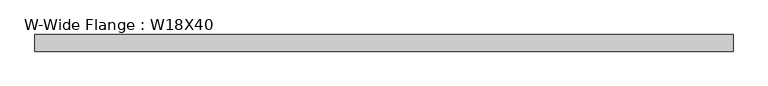
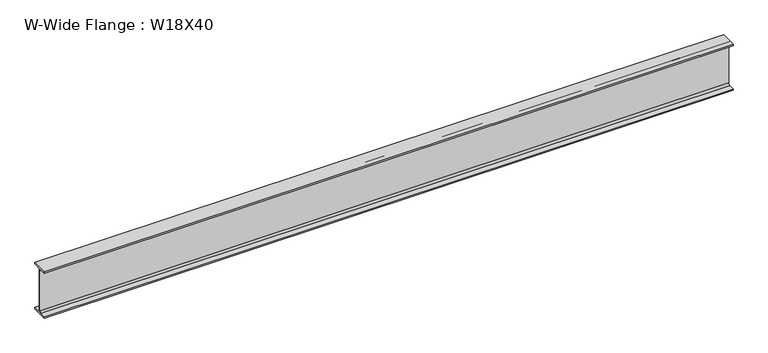
"""IFC4 building model written with IfcOpenShell, lengths in millimetres: beam geometry, W-Wide Flange : W18X40."""

import ifcopenshell
import ifcopenshell.guid

model = None  # the IFC model being written
_history = None  # IfcOwnerHistory: only IFC2X3 demands one
_inside = {}  # id of a spatial element -> (the spatial element, [elements in it])
_under = {}  # id of a project, library or spatial element -> (it, [spatial elements below it])
_declared = {}  # id of a project -> (the project, [libraries it declares])
_typed = {}  # id of a type object -> (the type object, [elements of that type])
_made_of = {}  # id of a material, layer set ... -> (it, [elements and type objects made of it])


def new_model(schema):
    """Start an empty IFC model of exactly this schema.

    Asked for "IFC4X3", IfcOpenShell would pick the latest addendum, in which some entities
    have other attributes; the version numbers below select the first issue.
    IFC2X3 requires an IfcOwnerHistory on every rooted entity: one is made here for all.
    """
    global model, _history
    if schema == "IFC4X3":
        model = ifcopenshell.file(schema_version=(4, 3, 0, 0))
    else:
        model = ifcopenshell.file(schema=schema)
    _inside.clear()
    _under.clear()
    _declared.clear()
    _typed.clear()
    _made_of.clear()
    _history = None
    if model.schema == "IFC2X3":
        org = make("IfcOrganization", Name="unknown")
        user = make(
            "IfcPersonAndOrganization",
            ThePerson=make("IfcPerson", FamilyName="unknown"),
            TheOrganization=org,
        )
        app = make(
            "IfcApplication",
            ApplicationDeveloper=org,
            Version="unknown",
            ApplicationFullName="unknown",
            ApplicationIdentifier="unknown",
        )
        _history = make(
            "IfcOwnerHistory",
            OwningUser=user,
            OwningApplication=app,
            ChangeAction="ADDED",
            CreationDate=0,
        )
    return model


def make(cls, **values):
    """One entity of the class cls with the attributes given. An attribute that is None is left unset."""
    return model.create_entity(
        cls, **{name: value for name, value in values.items() if value is not None}
    )


def rooted(cls, **values):
    """An entity with a GlobalId (a new one), such as an element, a storey or a relation."""
    return make(cls, GlobalId=ifcopenshell.guid.new(), OwnerHistory=_history, **values)


def si_unit(unit_type, name, prefix=None):
    """IfcSIUnit, for example si_unit("LENGTHUNIT", "METRE", prefix="MILLI")."""
    return make("IfcSIUnit", UnitType=unit_type, Prefix=prefix, Name=name)


def assignment(units):
    """IfcUnitAssignment: the units of a project."""
    return None if units is None else make("IfcUnitAssignment", Units=units)


def point(xyz):
    """IfcCartesianPoint."""
    return None if xyz is None else make("IfcCartesianPoint", Coordinates=xyz)


def direction(xyz):
    """IfcDirection."""
    return None if xyz is None else make("IfcDirection", DirectionRatios=xyz)


def frame(location, z_axis=None, x_axis=None):
    """IfcAxis2Placement3D, a coordinate frame: its origin and axes. An axis left out is left unset."""
    return make(
        "IfcAxis2Placement3D",
        Location=point(location),
        Axis=direction(z_axis),
        RefDirection=direction(x_axis),
    )


def frame_2d(location, x_axis=None):
    """IfcAxis2Placement2D, a coordinate frame in the plane: its origin and x axis."""
    return make(
        "IfcAxis2Placement2D", Location=point(location), RefDirection=direction(x_axis)
    )


def origin():
    """The frame at (0, 0, 0) with its axes left unset."""
    return frame((0.0, 0.0, 0.0))


def place(relative_to, where):
    """IfcLocalPlacement: puts the frame where relative to a parent placement (None: the world)."""
    return make(
        "IfcLocalPlacement", PlacementRelTo=relative_to, RelativePlacement=where
    )


def context(
    kind, dimensions, precision=None, world=None, true_north=None, identifier=None
):
    """IfcGeometricRepresentationContext, for example the 3D "Model" context."""
    return make(
        "IfcGeometricRepresentationContext",
        ContextIdentifier=identifier,
        ContextType=kind,
        CoordinateSpaceDimension=dimensions,
        Precision=precision,
        WorldCoordinateSystem=world,
        TrueNorth=true_north,
    )


def project(units=None, contexts=None):
    """IfcProject with its units and contexts."""
    return rooted(
        "IfcProject",
        Name="project",
        RepresentationContexts=contexts,
        UnitsInContext=assignment(units),
    )


def spatial(cls, under=None, at=None, **own):
    """A site, building, storey or space (cls), placed at a placement, below another one or the project."""
    s = rooted(cls, ObjectPlacement=at, **own)
    if under is not None:
        _under.setdefault(under.id(), (under, []))[1].append(s)
    return s


def polyline(points):
    """IfcPolyline through the points."""
    return make("IfcPolyline", Points=[point(p) for p in points])


def circle_curve(where, radius):
    """IfcCircle in the frame where."""
    return make("IfcCircle", Position=where, Radius=radius)


def trimmed(basis, trim1, trim2, sense, master):
    """IfcTrimmedCurve: the piece of a basis curve between two trims."""
    return make(
        "IfcTrimmedCurve",
        BasisCurve=basis,
        Trim1=trim1,
        Trim2=trim2,
        SenseAgreement=sense,
        MasterRepresentation=master,
    )


def segment(curve, same_sense, transition):
    """IfcCompositeCurveSegment."""
    return make(
        "IfcCompositeCurveSegment",
        Transition=transition,
        SameSense=same_sense,
        ParentCurve=curve,
    )


def composite_curve(segments, self_intersect=None):
    """IfcCompositeCurve: segments joined end to end."""
    return make("IfcCompositeCurve", Segments=segments, SelfIntersect=self_intersect)


def outline(outer, holes=None, kind="AREA"):
    """IfcArbitraryClosedProfileDef: a profile drawn as a closed curve; with holes, ...WithVoids."""
    if holes is None:
        return make("IfcArbitraryClosedProfileDef", ProfileType=kind, OuterCurve=outer)
    return make(
        "IfcArbitraryProfileDefWithVoids",
        ProfileType=kind,
        OuterCurve=outer,
        InnerCurves=holes,
    )


def extrude(swept, where, along, depth):
    """IfcExtrudedAreaSolid: the profile swept, set in the frame where, extruded along a direction by depth."""
    return make(
        "IfcExtrudedAreaSolid",
        SweptArea=swept,
        Position=where,
        ExtrudedDirection=direction(along),
        Depth=depth,
    )


def shape(context_of_items, identifier, shape_type, items):
    """IfcShapeRepresentation: the items that make up one representation, for example the "Body"."""
    return make(
        "IfcShapeRepresentation",
        ContextOfItems=context_of_items,
        RepresentationIdentifier=identifier,
        RepresentationType=shape_type,
        Items=items,
    )


def source(mapping_origin, context_of_items, identifier, shape_type, items):
    """IfcRepresentationMap: a shape defined once, which mapped items show again and again."""
    return make(
        "IfcRepresentationMap",
        MappingOrigin=mapping_origin,
        MappedRepresentation=shape(context_of_items, identifier, shape_type, items),
    )


def transform(
    local_origin,
    x_axis=None,
    y_axis=None,
    z_axis=None,
    scale=None,
    scale2=None,
    scale3=None,
    uniform=True,
):
    """IfcCartesianTransformationOperator3D, or its non-uniform kind. x_axis, y_axis, z_axis: its Axis1, 2, 3."""
    if uniform:
        return make(
            "IfcCartesianTransformationOperator3D",
            Axis1=direction(x_axis),
            Axis2=direction(y_axis),
            LocalOrigin=point(local_origin),
            Scale=scale,
            Axis3=direction(z_axis),
        )
    return make(
        "IfcCartesianTransformationOperator3DnonUniform",
        Axis1=direction(x_axis),
        Axis2=direction(y_axis),
        LocalOrigin=point(local_origin),
        Scale=scale,
        Axis3=direction(z_axis),
        Scale2=scale2,
        Scale3=scale3,
    )


def mapped(mapping_source, mapping_target):
    """IfcMappedItem: shows the shape of a source again, moved by a transform."""
    return make(
        "IfcMappedItem", MappingSource=mapping_source, MappingTarget=mapping_target
    )


def made_of(thing, what):
    """Note that an element or type object is made of a material, layer set ...; save() writes the relation."""
    if what is not None:
        _made_of.setdefault(what.id(), (what, []))[1].append(thing)
    return thing


def element(
    cls,
    number,
    at=None,
    inside=None,
    cuts=None,
    type_object=None,
    material=None,
    context=None,
    identifier="Body",
    shape_type=None,
    held_by="IfcProductDefinitionShape",
    body=None,
    shapes=None,
    **own,
):
    """One element of the class cls, such as IfcWall. Its Tag is "e" and its number.

    at: its placement. inside: the storey or other place that contains it. cuts: it is an
    opening in that element (IfcRelVoidsElement). A single representation is given by context,
    identifier, shape_type and body (its items); several are given by shapes. held_by: the class
    of the entity that holds the representations. save() writes the other relations.
    """
    e = rooted(cls, Tag="e%d" % number, ObjectPlacement=at, **own)
    if body is not None:
        shapes = [shape(context, identifier, shape_type, body)]
    if shapes is not None:
        e.Representation = make(held_by, Representations=shapes)
    if inside is not None:
        _inside.setdefault(inside.id(), (inside, []))[1].append(e)
    if cuts is not None:
        rooted(
            "IfcRelVoidsElement", RelatingBuildingElement=cuts, RelatedOpeningElement=e
        )
    if type_object is not None:
        _typed.setdefault(type_object.id(), (type_object, []))[1].append(e)
    return made_of(e, material)


def aggregate(whole, parts):
    """IfcRelAggregates: a whole, such as a stair, and the parts it consists of."""
    return rooted("IfcRelAggregates", RelatingObject=whole, RelatedObjects=parts)


def save(model, path):
    """Write the relations noted so far, then the file.

    IfcRelAggregates (storeys below a building ...), IfcRelContainedInSpatialStructure (elements
    in a storey), IfcRelDefinesByType, IfcRelAssociatesMaterial and IfcRelDeclares: one each for
    every whole, place, type object, material and project.
    """
    for whole, parts in _under.values():
        aggregate(whole, parts)
    for where, things in _inside.values():
        rooted(
            "IfcRelContainedInSpatialStructure",
            RelatedElements=things,
            RelatingStructure=where,
        )
    for kind, things in _typed.values():
        rooted("IfcRelDefinesByType", RelatedObjects=things, RelatingType=kind)
    for what, things in _made_of.values():
        rooted("IfcRelAssociatesMaterial", RelatedObjects=things, RelatingMaterial=what)
    for by, libraries in _declared.values():
        rooted("IfcRelDeclares", RelatingContext=by, RelatedDefinitions=libraries)
    model.write(path)


def w_wide_flange_w18x40_26c92dcf(model_context):
    return source(origin(), model_context, "Body", "SweptSolid", [
        extrude(outline(composite_curve([segment(polyline([(76.454, -213.995), (76.454, -227.33), (-76.454, -227.33), (-76.454, -213.995), (-20.828, -213.995)]), True, "CONTINUOUS"), segment(trimmed(circle_curve(frame_2d((-20.828, -197.1675)), 16.8275), [point((-20.828, -213.995))], [point((-4.0005, -197.1675))], True, "CARTESIAN"), True, "CONTINUOUS"), segment(polyline([(-4.0005, -197.1675), (-4.0005, 197.1675)]), True, "CONTINUOUS"), segment(trimmed(circle_curve(frame_2d((-20.828, 197.1675)), 16.8275), [point((-4.0005, 197.1675))], [point((-20.828, 213.995))], True, "CARTESIAN"), True, "CONTINUOUS"), segment(polyline([(-20.828, 213.995), (-76.454, 213.995), (-76.454, 227.33), (76.454, 227.33), (76.454, 213.995), (20.828, 213.995)]), True, "CONTINUOUS"), segment(trimmed(circle_curve(frame_2d((20.828, 197.1675)), 16.8275), [point((20.828, 213.995))], [point((4.0005, 197.1675))], True, "CARTESIAN"), True, "CONTINUOUS"), segment(polyline([(4.0005, 197.1675), (4.0005, -197.1675)]), True, "CONTINUOUS"), segment(trimmed(circle_curve(frame_2d((20.828, -197.1675)), 16.8275), [point((4.0005, -197.1675))], [point((20.828, -213.995))], True, "CARTESIAN"), True, "CONTINUOUS"), segment(polyline([(20.828, -213.995), (76.454, -213.995)]), True, "CONTINUOUS")], self_intersect=False)), frame((-3211.83, 0.0, 0.0), z_axis=(1.0, 0.0, 0.0), x_axis=(0.0, 1.0, 0.0)), (0.0, 0.0, 1.0), 6418.58),
    ])


if __name__ == "__main__":
    model = new_model("IFC4")
    model_context = context("Model", 3, world=origin())
    ifc_project = project(units=[si_unit("LENGTHUNIT", "METRE", prefix="MILLI")], contexts=[model_context])
    site = spatial("IfcSite", under=ifc_project)
    building = spatial("IfcBuilding", under=site)
    placement = place(None, origin())
    w_wide_flange_w18x40_shape = w_wide_flange_w18x40_26c92dcf(model_context)
    element("IfcBeam", 1, ObjectType="W-Wide Flange : W18X40", at=placement, inside=building, context=model_context, shape_type="MappedRepresentation", body=[
        mapped(w_wide_flange_w18x40_shape, transform((0.0, 0.0, 0.0), x_axis=(1.0, 0.0, 0.0), y_axis=(0.0, 1.0, 0.0), z_axis=(0.0, 0.0, 1.0))),
    ])
    save(model, "model.ifc")

# Revit data of these elements
# Type "W-Wide Flange : W18X40"
#   Assembly Code = "B10"
#   W = 40
#   Length [instance default] = 5' - 0"
#   bf = 0' - 6.02"
#   d = 1' - 5.9"
#   k = 0' - 1 3/16"
#   k2 = 0' - 0.6625"
#   tf = 0' - 0.525"
#   tw = 0' - 0.315"
#   A = 0.0819444 SF
#   Structural Material [instance default] = Steel ASTM A992
# Element 1 (IfcBeam, "W-Wide Flange : W18X40")
#   Materials on its faces: "Steel ASTM A992"
# Materials
#   "Steel ASTM A992": class "Metal", colour RGB 199 199 199, transparency 0, Description = "Structural steel 50ksi", Cost = 0
